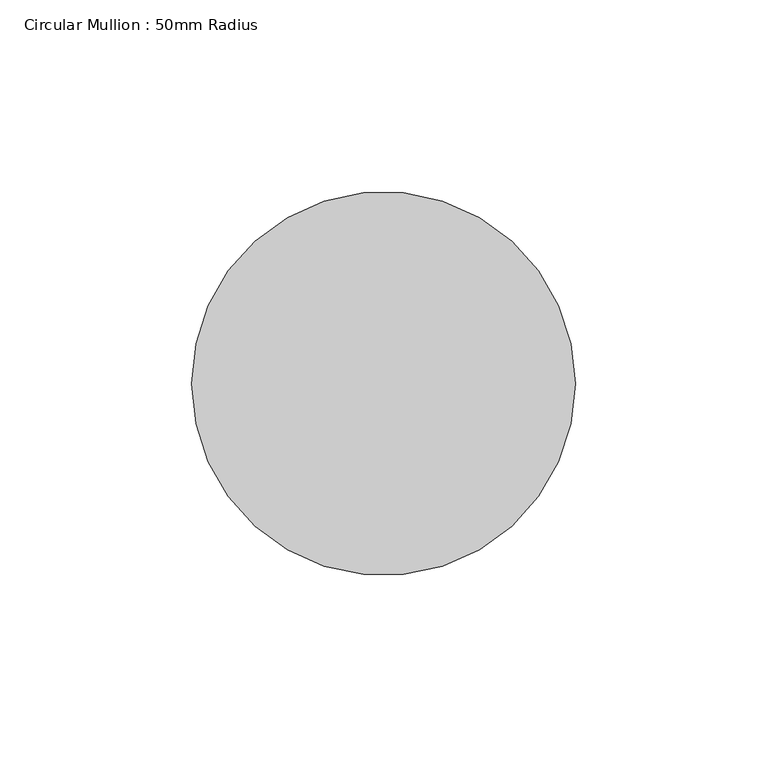
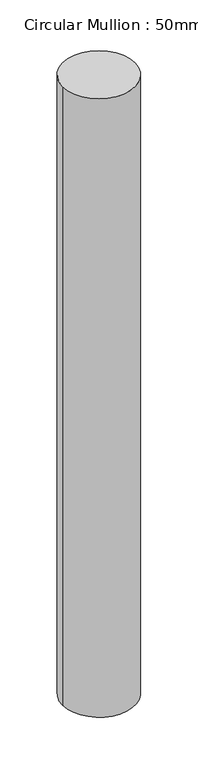
"""IFC4 building model written with IfcOpenShell, lengths in millimetres: member geometry, Circular Mullion : 50mm Radius."""

from ifc_helpers import new_model, si_unit, point, frame, origin, origin_2d, place, context, project, spatial, circle_curve, trimmed, segment, composite_curve, outline, extrude, source, transform, mapped, element, save


def circular_mullion_50mm_radius_2fdd6397(model_context):
    return source(origin(), model_context, "Body", "SweptSolid", [
        extrude(outline(composite_curve([segment(trimmed(circle_curve(origin_2d(), 50.0), [point((50.0, 0.0))], [point((-50.0, 0.0))], False, "CARTESIAN"), True, "CONTINUOUS"), segment(trimmed(circle_curve(origin_2d(), 50.0), [point((-50.0, 0.0))], [point((50.0, 0.0))], False, "CARTESIAN"), True, "CONTINUOUS")], self_intersect=False)), frame((0.0, 0.0, -901.1789241), z_axis=(0.0, 0.0, 1.0), x_axis=(1.0, 0.0, 0.0)), (0.0, 0.0, 1.0), 901.1789241),
    ])


if __name__ == "__main__":
    model = new_model("IFC4")
    model_context = context("Model", 3, world=origin())
    ifc_project = project(units=[si_unit("LENGTHUNIT", "METRE", prefix="MILLI")], contexts=[model_context])
    site = spatial("IfcSite", under=ifc_project)
    building = spatial("IfcBuilding", under=site)
    placement = place(None, origin())
    circular_mullion_50mm_radius_shape = circular_mullion_50mm_radius_2fdd6397(model_context)
    element("IfcMember", 1, ObjectType="Circular Mullion : 50mm Radius", at=placement, inside=building, context=model_context, shape_type="MappedRepresentation", body=[
        mapped(circular_mullion_50mm_radius_shape, transform((0.0, 0.0, 0.0), x_axis=(1.0, 0.0, 0.0), y_axis=(0.0, 1.0, 0.0), z_axis=(0.0, 0.0, 1.0))),
    ])
    save(model, "model.ifc")

# Revit data of these elements
# Type "Circular Mullion : 50mm Radius"
#   built-in parameter 1007350 = 0.164042 (stored number, unit not read)
# Element 1 (IfcMember, "Circular Mullion : 50mm Radius")
#   Materials on its faces: "Aluminium"
# Materials
#   "Aluminium": class "Metal", colour RGB 247 247 247, transparency 0, Description = "Aluminium 6061", Cost = 0
